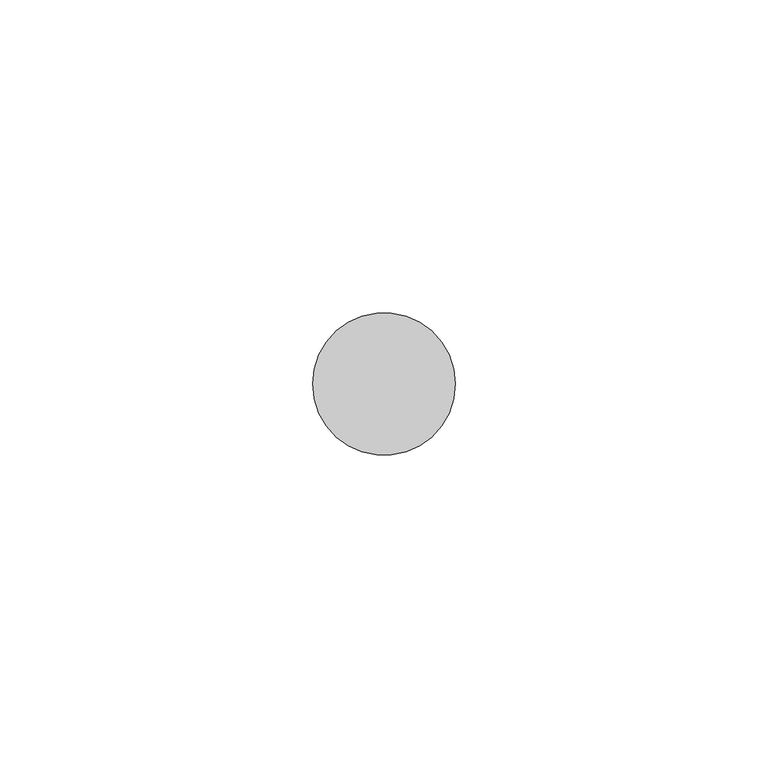
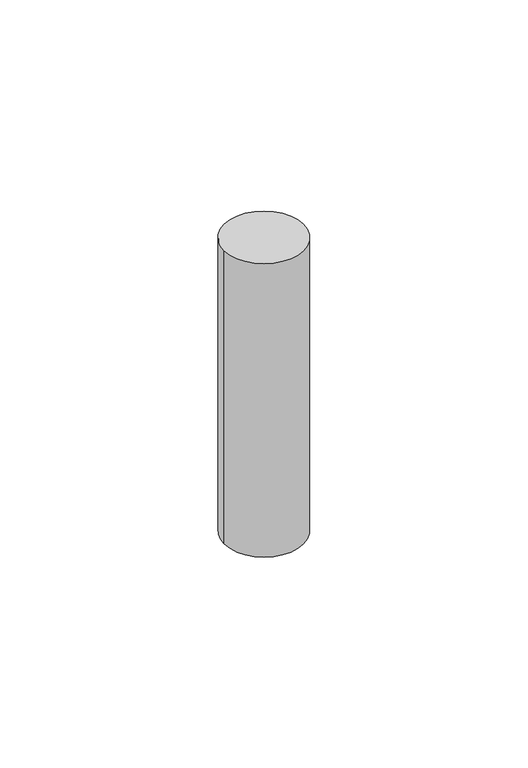
"""IFC4 building model written with IfcOpenShell, lengths in millimetres: proxy geometry, Bolt9:Bolt003:304204 : Bolt9:Bolt003:304204."""

from ifc_helpers import new_model, si_unit, point, frame, frame_2d, origin, place, context, project, spatial, circle_curve, trimmed, segment, composite_curve, outline, extrude, source, transform, mapped, element, save


def generic_models_0fd4d913(model_context):
    return source(origin(), model_context, "Body", "SweptSolid", [
        extrude(outline(composite_curve([segment(trimmed(circle_curve(frame_2d((9923.9919204, 2174.9207483)), 11.4045168), [point((9912.5874035, 2174.9207483))], [point((9935.3964372, 2174.9207483))], False, "CARTESIAN"), True, "CONTINUOUS"), segment(trimmed(circle_curve(frame_2d((9923.9919204, 2174.9207483)), 11.4045168), [point((9935.3964372, 2174.9207483))], [point((9912.5874035, 2174.9207483))], False, "CARTESIAN"), True, "CONTINUOUS")], self_intersect=False)), frame((0.0, 0.0, 36645.5959962), z_axis=(0.0, 0.0, 1.0), x_axis=(1.0, 0.0, 0.0)), (0.0, 0.0, 1.0), 88.9),
    ])


if __name__ == "__main__":
    model = new_model("IFC4")
    model_context = context("Model", 3, world=origin())
    ifc_project = project(units=[si_unit("LENGTHUNIT", "METRE", prefix="MILLI")], contexts=[model_context])
    site = spatial("IfcSite", under=ifc_project)
    building = spatial("IfcBuilding", under=site)
    placement = place(None, origin())
    generic_models_shape = generic_models_0fd4d913(model_context)
    element("IfcBuildingElementProxy", 1, Name="Bolt9:Bolt003:304204 : Bolt9:Bolt003:304204", ObjectType="Bolt9:Bolt003:304204 : Bolt9:Bolt003:304204", at=placement, inside=building, context=model_context, shape_type="MappedRepresentation", body=[
        mapped(generic_models_shape, transform((0.0, 0.0, 0.0), x_axis=(1.0, 0.0, 0.0), y_axis=(0.0, 1.0, 0.0), z_axis=(0.0, 0.0, 1.0))),
    ])
    save(model, "model.ifc")

# Revit data of these elements
# Type "Bolt9:Bolt003:304204 : Bolt9:Bolt003:304204"
#   NameOverride = "Bolt9:Bolt003:304204"
#   ObjectTypeOverride = "Bolt9:Bolt003"
#   Reference = "Bolt003"
#   Category = "Generic Models"
#   Tag = "304204"
# Element 1 (IfcBuildingElementProxy, "Bolt9:Bolt003:304204 : Bolt9:Bolt003:304204")
#   Materials on its faces: "TUBE STEEL STRINGER WELDED TO ANCHORED STEEL PLATE - SEE STRUCT DWGS"
# Materials
#   "TUBE STEEL STRINGER WELDED TO ANCHORED STEEL PLATE - SEE STRUCT DWGS": class "Unassigned", colour RGB 128 128 128, transparency 0, Cost = 0
